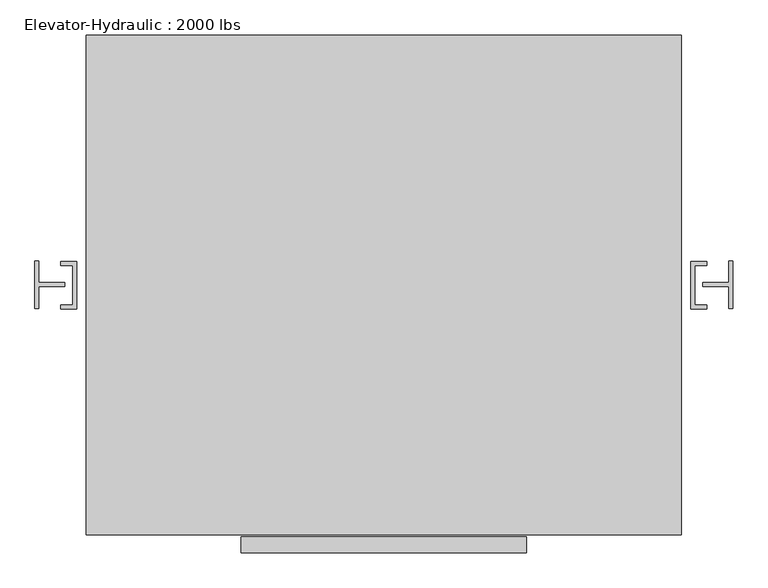
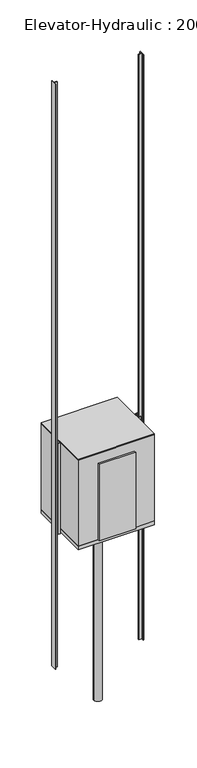
"""IFC4 building model written with IfcOpenShell, lengths in millimetres: proxy geometry, Elevator-Hydraulic : 2000 lbs."""

from ifc_helpers import new_model, si_unit, point, frame, frame_2d, origin, origin_with_axes, place, context, project, spatial, polyline, circle_curve, trimmed, segment, composite_curve, outline, extrude, faceted_brep, source, transform, mapped, element, save


def elevator_hydraulic_2000_lbs_0253a703(model_context):
    return source(origin(), model_context, "Body", "SolidModel", [
        faceted_brep([(-945.0530035, -797.2781737, 5943.6), (959.9469965, -797.2781737, 5943.6), (959.9469965, 802.9218263, 5943.6), (-945.0530035, 802.9218263, 5943.6), (921.8469965, 764.8218263, 5943.6), (921.8469965, -759.1781737, 5943.6), (-906.9530035, -759.1781737, 5943.6), (-906.9530035, 764.8218263, 5943.6), (-906.9530035, 764.8218263, 3657.6), (-906.9530035, -759.1781737, 3657.6), (-449.7530035, -759.1781737, 3657.6), (-449.7530035, -797.2781737, 3657.6), (-945.0530035, -797.2781737, 3657.6), (-945.0530035, 802.9218263, 3657.6), (959.9469965, 802.9218263, 3657.6), (959.9469965, -797.2781737, 3657.6), (464.6469965, -797.2781737, 3657.6), (464.6469965, -759.1781737, 3657.6), (921.8469965, -759.1781737, 3657.6), (921.8469965, 764.8218263, 3657.6), (464.6469965, 764.8218263, 3657.6), (-449.7530035, 764.8218263, 3657.6), (464.6469965, -759.1781737, 5689.6), (-449.7530035, -759.1781737, 5689.6), (-449.7530035, -797.2781737, 5689.6), (464.6469965, -797.2781737, 5689.6)], [[[0, 1, 2, 3], [4, 5, 6, 7]], [[8, 9, 10, 11, 12, 13, 14, 15, 16, 17, 18, 19, 20, 21]], [[5, 4, 19, 18]], [[6, 5, 18, 17, 22, 23, 10, 9]], [[7, 6, 9, 8]], [[4, 7, 8, 21, 20, 19]], [[1, 0, 12, 11, 24, 25, 16, 15]], [[2, 1, 15, 14]], [[3, 2, 14, 13]], [[0, 3, 13, 12]], [[22, 25, 24, 23]], [[23, 24, 11, 10]], [[25, 22, 17, 16]]]),
        extrude(outline(polyline([(464.6469965, -803.6281737), (464.6469965, -854.4281737), (-449.7530035, -854.4281737), (-449.7530035, -803.6281737), (464.6469965, -803.6281737)])), frame((0.0, 0.0, 3657.6), z_axis=(0.0, 0.0, 1.0), x_axis=(1.0, 0.0, 0.0)), (0.0, 0.0, 1.0), 2032.0),
        extrude(outline(polyline([(959.9469965, 802.9218263), (959.9469965, -797.2781737), (-945.0530035, -797.2781737), (-945.0530035, 802.9218263), (959.9469965, 802.9218263)])), frame((0.0, 0.0, 5943.6), z_axis=(0.0, 0.0, 1.0), x_axis=(1.0, 0.0, 0.0)), (0.0, 0.0, 1.0), 25.4),
        extrude(outline(composite_curve([segment(trimmed(circle_curve(frame_2d((7.4469965, 2.8218263)), 101.6), [point((-94.1530035, 2.8218263))], [point((109.0469965, 2.8218263))], False, "CARTESIAN"), True, "CONTINUOUS"), segment(trimmed(circle_curve(frame_2d((7.4469965, 2.8218263)), 101.6), [point((109.0469965, 2.8218263))], [point((-94.1530035, 2.8218263))], False, "CARTESIAN"), True, "CONTINUOUS")], self_intersect=False)), frame((0.0, 0.0, -1219.2), z_axis=(0.0, 0.0, 1.0), x_axis=(1.0, 0.0, 0.0)), (0.0, 0.0, 1.0), 4775.2),
        extrude(outline(polyline([(959.9469965, 802.9218263), (959.9469965, -797.2781737), (-945.0530035, -797.2781737), (-945.0530035, 802.9218263), (959.9469965, 802.9218263)])), frame((0.0, 0.0, 3556.0), z_axis=(0.0, 0.0, 1.0), x_axis=(1.0, 0.0, 0.0)), (0.0, 0.0, 1.0), 101.6),
        extrude(outline(polyline([(-976.8030035, 79.0218263), (-976.8030035, -73.3781737), (-1027.6030035, -73.3781737), (-1027.6030035, -60.6781737), (-989.5030035, -60.6781737), (-989.5030035, 66.3218263), (-1027.6030035, 66.3218263), (-1027.6030035, 79.0218263), (-976.8030035, 79.0218263)])), frame((0.0, 0.0, 3556.0), z_axis=(0.0, 0.0, 1.0), x_axis=(1.0, 0.0, 0.0)), (0.0, 0.0, 1.0), 2413.0),
        extrude(outline(polyline([(991.6969965, 79.0218263), (1042.4969965, 79.0218263), (1042.4969965, 66.3218263), (1004.3969965, 66.3218263), (1004.3969965, -60.6781737), (1042.4969965, -60.6781737), (1042.4969965, -73.3781737), (991.6969965, -73.3781737), (991.6969965, 79.0218263)])), frame((0.0, 0.0, 3556.0), z_axis=(0.0, 0.0, 1.0), x_axis=(1.0, 0.0, 0.0)), (0.0, 0.0, 1.0), 2413.0),
        extrude(outline(polyline([(-1097.4530035, 79.0218263), (-1097.4530035, 9.1718263), (-1014.9030035, 9.1718263), (-1014.9030035, -3.5281737), (-1097.4530035, -3.5281737), (-1097.4530035, -73.3781737), (-1110.1530035, -73.3781737), (-1110.1530035, 79.0218263), (-1097.4530035, 79.0218263)])), origin_with_axes(), (0.0, 0.0, 1.0), 15544.8),
        extrude(outline(polyline([(1112.3469965, 79.0218263), (1125.0469965, 79.0218263), (1125.0469965, -73.3781737), (1112.3469965, -73.3781737), (1112.3469965, -3.5281737), (1029.7969965, -3.5281737), (1029.7969965, 9.1718263), (1112.3469965, 9.1718263), (1112.3469965, 79.0218263)])), origin_with_axes(), (0.0, 0.0, 1.0), 15544.8),
    ])


if __name__ == "__main__":
    model = new_model("IFC4")
    model_context = context("Model", 3, world=origin())
    ifc_project = project(units=[si_unit("LENGTHUNIT", "METRE", prefix="MILLI")], contexts=[model_context])
    site = spatial("IfcSite", under=ifc_project)
    building = spatial("IfcBuilding", under=site)
    placement = place(None, origin())
    elevator_hydraulic_2000_lbs_shape = elevator_hydraulic_2000_lbs_0253a703(model_context)
    element("IfcBuildingElementProxy", 1, Name="Elevator-Hydraulic : 2000 lbs", ObjectType="Elevator-Hydraulic : 2000 lbs", at=placement, inside=building, context=model_context, shape_type="MappedRepresentation", body=[
        mapped(elevator_hydraulic_2000_lbs_shape, transform((0.0, 0.0, 0.0), x_axis=(1.0, 0.0, 0.0), y_axis=(0.0, 1.0, 0.0), z_axis=(0.0, 0.0, 1.0))),
    ])
    save(model, "model.ifc")

# Revit data of these elements
# Project information
#   Organization Name = "G3B Press"
#   Organization Description = "Paul F. Aubin Cosulting Services, Inc."
#   Building Name = "Revit Essentials for Architecture"
#   Author = "Paul F. Aubin"
#   Author Website = "https://www.paulaubin.com"
#   Copyright = "Copyright © 2020 Paul F Aubin, all rights reserved"
#   Project Issue Date = "8/1/2020"
#   Project Status = "Design Development"
#   Client Name = "Vertical Circulation"
#   Project Address = "123 State ST\nSuite 301\nChicago, IL 60606"
#   Project Name = "08 Commercial_Complete"
#   Project Number = "2020.04A"
# Type "Elevator-Hydraulic : 2000 lbs"
#   Cab Location = 12' - 0"
#   Width = 7' - 4"
#   Pit Depth = 4' - 0"
#   Height [instance default] = 36' - 0"
#   Door Opening = 3' - 0"
#   Depth = 5' - 9"
#   Cab Width = 6' - 0"
#   Cab Height = 7' - 6"
#   Cab Depth = 5' - 0"
#   Default Elevation = 0
# Element 1 (IfcBuildingElementProxy, "Elevator-Hydraulic : 2000 lbs")
#   Height = 51' - 0"
#   Materials on its faces: "Metal - Steel"
# Materials
#   "Metal - Steel": class "Metal", colour RGB 247 247 247, transparency 0
